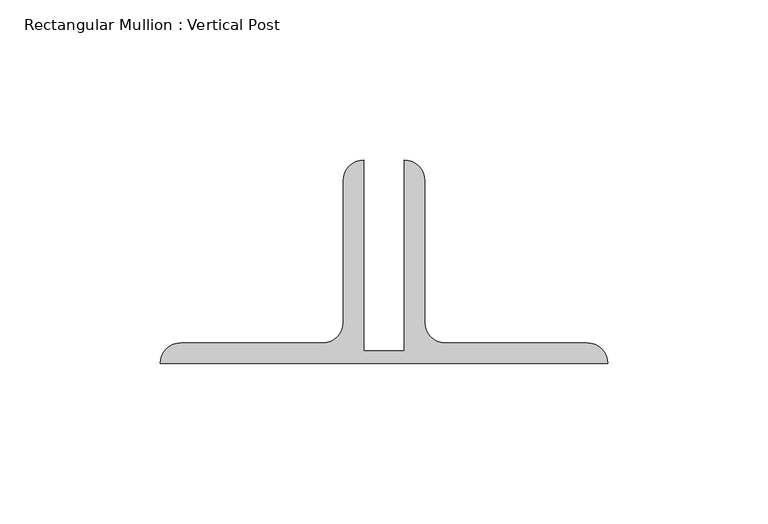
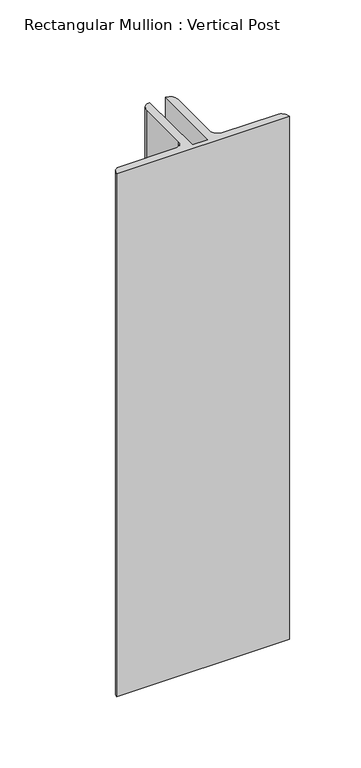
"""IFC4 building model written with IfcOpenShell, lengths in millimetres: member geometry, Rectangular Mullion : Vertical Post."""

from ifc_helpers import new_model, si_unit, point, frame, frame_2d, origin, place, context, project, spatial, polyline, circle_curve, trimmed, segment, composite_curve, outline, extrude, source, transform, mapped, element, save


def rectangular_mullion_vertical_post_4fcf061c(model_context):
    return source(origin(), model_context, "Body", "SweptSolid", [
        extrude(outline(composite_curve([segment(polyline([(-6.35, 22.9145205), (6.35, 22.9145205), (6.35, 82.55)]), True, "CONTINUOUS"), segment(trimmed(circle_curve(frame_2d((6.35, 76.2)), 6.35), [point((6.35, 82.55))], [point((12.7, 76.2))], False, "CARTESIAN"), True, "CONTINUOUS"), segment(polyline([(12.7, 76.2), (12.7, 31.75)]), True, "CONTINUOUS"), segment(trimmed(circle_curve(frame_2d((19.05, 31.75)), 6.35), [point((12.7, 31.75))], [point((19.05, 25.4))], True, "CARTESIAN"), True, "CONTINUOUS"), segment(polyline([(19.05, 25.4), (63.5, 25.4)]), True, "CONTINUOUS"), segment(trimmed(circle_curve(frame_2d((63.5, 19.05)), 6.35), [point((63.5, 25.4))], [point((69.85, 19.05))], False, "CARTESIAN"), True, "CONTINUOUS"), segment(polyline([(69.85, 19.05), (-69.85, 19.05)]), True, "CONTINUOUS"), segment(trimmed(circle_curve(frame_2d((-63.5, 19.05)), 6.35), [point((-69.85, 19.05))], [point((-63.5, 25.4))], False, "CARTESIAN"), True, "CONTINUOUS"), segment(polyline([(-63.5, 25.4), (-19.05, 25.4)]), True, "CONTINUOUS"), segment(trimmed(circle_curve(frame_2d((-19.05, 31.75)), 6.35), [point((-19.05, 25.4))], [point((-12.7, 31.75))], True, "CARTESIAN"), True, "CONTINUOUS"), segment(polyline([(-12.7, 31.75), (-12.7, 76.2)]), True, "CONTINUOUS"), segment(trimmed(circle_curve(frame_2d((-6.35, 76.2)), 6.35), [point((-12.7, 76.2))], [point((-6.35, 82.55))], False, "CARTESIAN"), True, "CONTINUOUS"), segment(polyline([(-6.35, 82.55), (-6.35, 22.9145205)]), True, "CONTINUOUS")], self_intersect=False)), frame((0.0, 0.0, -446.7663052), z_axis=(0.0, 0.0, 1.0), x_axis=(1.0, 0.0, 0.0)), (0.0, 0.0, 1.0), 446.7663052),
    ])


if __name__ == "__main__":
    model = new_model("IFC4")
    model_context = context("Model", 3, world=origin())
    ifc_project = project(units=[si_unit("LENGTHUNIT", "METRE", prefix="MILLI")], contexts=[model_context])
    site = spatial("IfcSite", under=ifc_project)
    building = spatial("IfcBuilding", under=site)
    placement = place(None, origin())
    rectangular_mullion_vertical_post_shape = rectangular_mullion_vertical_post_4fcf061c(model_context)
    element("IfcMember", 1, ObjectType="Rectangular Mullion : Vertical Post", at=placement, inside=building, context=model_context, shape_type="MappedRepresentation", body=[
        mapped(rectangular_mullion_vertical_post_shape, transform((0.0, 0.0, 0.0), x_axis=(1.0, 0.0, 0.0), y_axis=(0.0, 1.0, 0.0), z_axis=(0.0, 0.0, 1.0))),
    ])
    save(model, "model.ifc")

# Revit data of these elements
# Type "Rectangular Mullion : Vertical Post"
#   built-in parameter 1007351 = -0.0625 (stored number, unit not read)
#   built-in parameter 1007322 = 0.0126789 (stored number, unit not read)
#   built-in parameter 1007321 = 0.229167 (stored number, unit not read)
#   built-in parameter 1007320 = 0.229167 (stored number, unit not read)
# Element 1 (IfcMember, "Rectangular Mullion : Vertical Post")
#   Materials on its faces: "GATE POST: GALVANIZED ANGLES"
# Materials
#   "GATE POST: GALVANIZED ANGLES": class "Unassigned", colour RGB 211 211 211, transparency 0, Cost = 0
